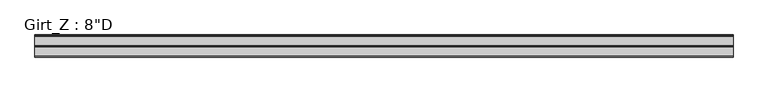
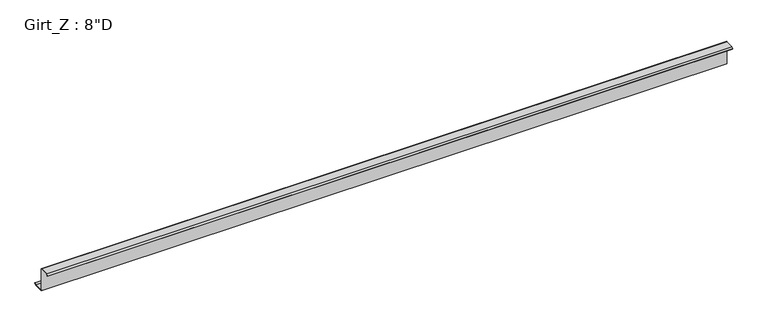
"""IFC4 building model written with IfcOpenShell, lengths in millimetres: beam geometry."""

from ifc_helpers import new_model, si_unit, point, frame, frame_2d, origin, place, context, project, spatial, polyline, circle_curve, trimmed, segment, composite_curve, outline, extrude, source, transform, mapped, element, save


def beam_fa2c950f(model_context):
    return source(origin(), model_context, "Body", "SweptSolid", [
        extrude(outline(composite_curve([segment(polyline([(-77.9859375, 101.6), (-3.3734375, 101.6)]), True, "CONTINUOUS"), segment(trimmed(circle_curve(frame_2d((-3.3734375, 96.8375)), 4.7625), [point((-3.3734375, 101.6))], [point((1.3890625, 96.8375))], False, "CARTESIAN"), True, "CONTINUOUS"), segment(polyline([(1.3890625, 96.8375), (1.3890625, -96.8389339)]), True, "CONTINUOUS"), segment(trimmed(circle_curve(frame_2d((3.3748024, -96.8389339)), 1.9857399), [point((1.3890625, -96.8389339))], [point((3.2694106, -98.821875))], True, "CARTESIAN"), True, "CONTINUOUS"), segment(polyline([(3.2694106, -98.821875), (83.0404765, -98.821875), (94.4528742, -85.221109), (96.5810415, -87.0068534), (84.3359375, -101.6), (-1.3890625, -101.6), (-1.3890625, 96.8381931)]), True, "CONTINUOUS"), segment(trimmed(circle_curve(frame_2d((-3.3741066, 96.8381931)), 1.9850441), [point((-1.3890625, 96.8381931))], [point((-3.3005807, 98.821875))], True, "CARTESIAN"), True, "CONTINUOUS"), segment(polyline([(-3.3005807, 98.821875), (-76.6904765, 98.821875), (-88.1028742, 85.221109), (-90.2310415, 87.0068534), (-77.9859375, 101.6)]), True, "CONTINUOUS")], self_intersect=False)), frame((-2974.2892, 0.0, 0.0), z_axis=(1.0, 0.0, 0.0), x_axis=(0.0, 1.0, 0.0)), (0.0, 0.0, 1.0), 5890.514),
    ])


if __name__ == "__main__":
    model = new_model("IFC4")
    model_context = context("Model", 3, world=origin())
    ifc_project = project(units=[si_unit("LENGTHUNIT", "METRE", prefix="MILLI")], contexts=[model_context])
    site = spatial("IfcSite", under=ifc_project)
    building = spatial("IfcBuilding", under=site)
    placement = place(None, origin())
    beam_shape = beam_fa2c950f(model_context)
    element("IfcBeam", 1, ObjectType="Girt_Z : 8\"D", at=placement, inside=building, context=model_context, shape_type="MappedRepresentation", body=[
        mapped(beam_shape, transform((0.0, 0.0, 0.0), x_axis=(1.0, 0.0, 0.0), y_axis=(0.0, 1.0, 0.0), z_axis=(0.0, 0.0, 1.0))),
    ])
    save(model, "model.ifc")

# Revit data of these elements
# Type "Girt_Z : 8\"D"
#   half leg = 0' - 1 11/16"
#   Web_Thickness = 0' - 0 7/64"
#   Length [instance default] = 10' - 0"
#   Leg_2 = 0' - 3 3/8"
#   Leg_1 = 0' - 3 1/8"
#   Height = 0' - 8"
#   Structural Material [instance default] = none
